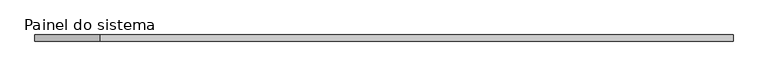
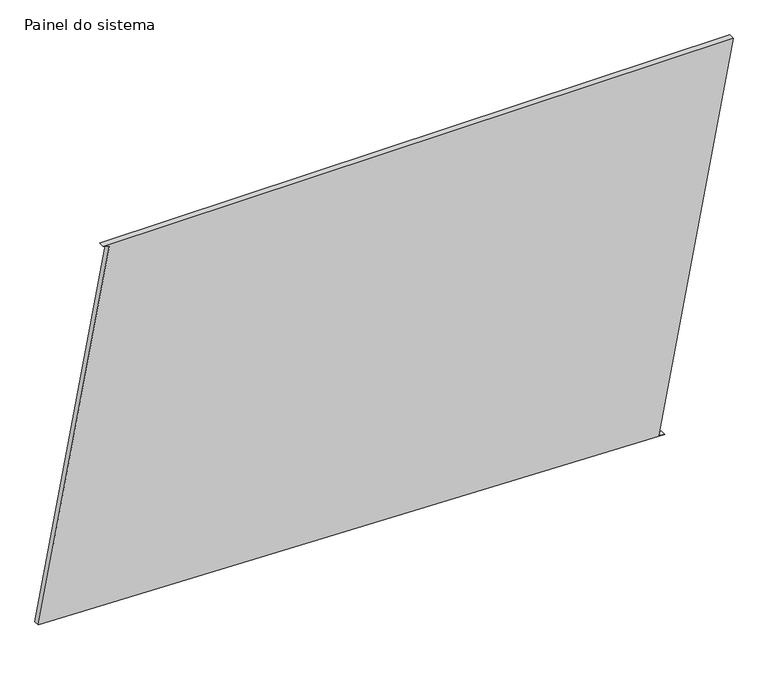
"""IFC4 building model written with IfcOpenShell, lengths in millimetres: plate geometry, Painel do sistema : Envidraçado."""

from ifc_helpers import new_model, si_unit, frame, origin, place, context, project, spatial, polyline, outline, extrude, source, transform, mapped, element, save


def painel_do_sistema_5d1635f8(model_context):
    return source(origin(), model_context, "Body", "SweptSolid", [
        extrude(outline(polyline([(0.0, 1148.9206839), (4.6288169, 1124.3529398), (1626.3532892, 1429.9025897), (1626.3532892, -1162.5504651), (1621.7244723, -1137.9827209), (72.3409423, -1429.9025897), (0.0, 1148.9206839)])), frame((0.0, 24.5, 0.0), z_axis=(0.0, 1.0, 0.0), x_axis=(0.0, 0.0, 1.0)), (0.0, 0.0, 1.0), 25.0),
    ])


if __name__ == "__main__":
    model = new_model("IFC4")
    model_context = context("Model", 3, world=origin())
    ifc_project = project(units=[si_unit("LENGTHUNIT", "METRE", prefix="MILLI")], contexts=[model_context])
    site = spatial("IfcSite", under=ifc_project)
    building = spatial("IfcBuilding", under=site)
    placement = place(None, origin())
    painel_do_sistema_shape = painel_do_sistema_5d1635f8(model_context)
    element("IfcPlate", 1, ObjectType="Painel do sistema : Envidraçado", at=placement, inside=building, context=model_context, shape_type="MappedRepresentation", body=[
        mapped(painel_do_sistema_shape, transform((0.0, 0.0, 0.0), x_axis=(1.0, 0.0, 0.0), y_axis=(0.0, 1.0, 0.0), z_axis=(0.0, 0.0, 1.0))),
    ])
    save(model, "model.ifc")

# Revit data of these elements
# Type "Painel do sistema : Envidraçado"
#   Construction Type Id = "GSP4R"
#   Analytic Construction = "Vidraça única Pilkington 1/8 pol"
#   Visual Light Transmittance = 0.9
#   Solar Heat Gain Coefficient = 0.86
#   Heat Transfer Coefficient (U) = 6.7069 W/(m²·K)
# Element 1 (IfcPlate, "Painel do sistema : Envidraçado")
#   Materials on its faces: "Vidro"
# Materials
#   "Vidro": class "Vidro", colour RGB 0 128 192, transparency 0.9, Description = "Vidro de sílica", Cost = 0
